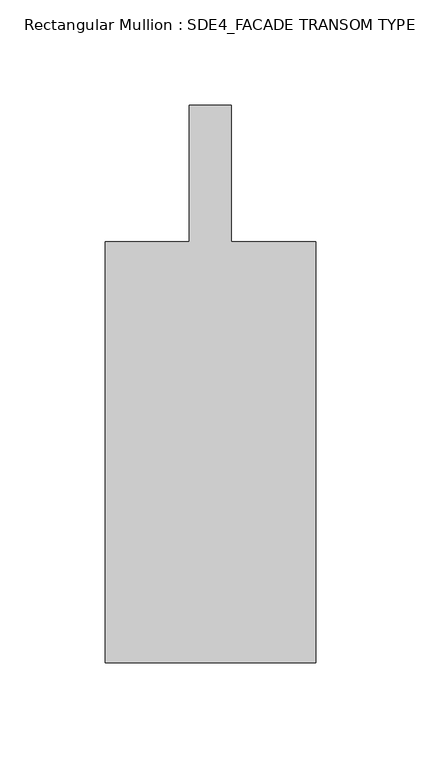
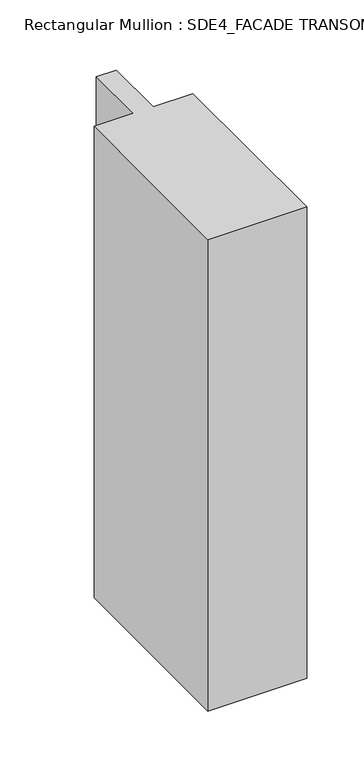
"""IFC4 building model written with IfcOpenShell, lengths in millimetres: member geometry, Rectangular Mullion : SDE4_FACADE TRANSOM TYPE 2."""

from ifc_helpers import new_model, si_unit, frame, origin, place, context, project, spatial, polyline, outline, extrude, source, transform, mapped, element, save


def rectangular_mullion_sde4_facade_transom_type_2_76915716(model_context):
    return source(origin(), model_context, "Body", "SweptSolid", [
        extrude(outline(polyline([(50.0, -132.5), (-50.0, -132.5), (-50.0, 67.5), (-10.0, 67.5), (-10.0, 132.5), (10.0, 132.5), (10.0, 67.5), (50.0, 67.5), (50.0, -132.5)])), frame((0.0, 0.0, -505.06364), z_axis=(0.0, 0.0, 1.0), x_axis=(1.0, 0.0, 0.0)), (0.0, 0.0, 1.0), 505.06364),
    ])


if __name__ == "__main__":
    model = new_model("IFC4")
    model_context = context("Model", 3, world=origin())
    ifc_project = project(units=[si_unit("LENGTHUNIT", "METRE", prefix="MILLI")], contexts=[model_context])
    site = spatial("IfcSite", under=ifc_project)
    building = spatial("IfcBuilding", under=site)
    placement = place(None, origin())
    rectangular_mullion_sde4_facade_transom_type_2_shape = rectangular_mullion_sde4_facade_transom_type_2_76915716(model_context)
    element("IfcMember", 1, ObjectType="Rectangular Mullion : SDE4_FACADE TRANSOM TYPE 2", at=placement, inside=building, context=model_context, shape_type="MappedRepresentation", body=[
        mapped(rectangular_mullion_sde4_facade_transom_type_2_shape, transform((0.0, 0.0, 0.0), x_axis=(1.0, 0.0, 0.0), y_axis=(0.0, 1.0, 0.0), z_axis=(0.0, 0.0, 1.0))),
    ])
    save(model, "model.ifc")

# Revit data of these elements
# Type "Rectangular Mullion : SDE4_FACADE TRANSOM TYPE 2"
#   built-in parameter 1007322 = 0.869423 (stored number, unit not read)
#   built-in parameter 1007321 = 0.164042 (stored number, unit not read)
#   built-in parameter 1007320 = 0.164042 (stored number, unit not read)
